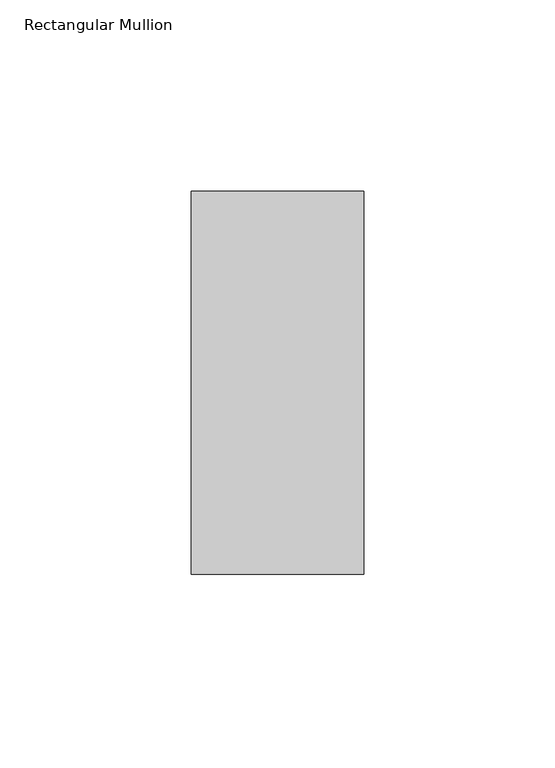
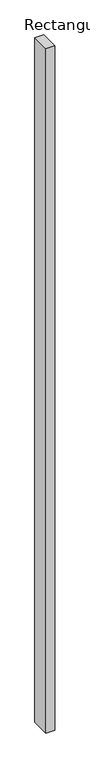
"""IFC4 building model written with IfcOpenShell, lengths in millimetres: member geometry, Rectangular Mullion : 알루미늄_Rectangular Cap_100 x 45."""

from ifc_helpers import new_model, si_unit, frame, origin, place, context, project, spatial, polyline, outline, extrude, source, transform, mapped, element, save


def rectangular_mullion_03c4161e(model_context):
    return source(origin(), model_context, "Body", "SweptSolid", [
        extrude(outline(polyline([(0.0, 50.0), (0.0, -50.0), (-45.0, -50.0), (-45.0, 50.0), (0.0, 50.0)])), frame((0.0, 0.0, -3775.0), z_axis=(0.0, 0.0, 1.0), x_axis=(1.0, 0.0, 0.0)), (0.0, 0.0, 1.0), 3775.0),
    ])


if __name__ == "__main__":
    model = new_model("IFC4")
    model_context = context("Model", 3, world=origin())
    ifc_project = project(units=[si_unit("LENGTHUNIT", "METRE", prefix="MILLI")], contexts=[model_context])
    site = spatial("IfcSite", under=ifc_project)
    building = spatial("IfcBuilding", under=site)
    placement = place(None, origin())
    rectangular_mullion_shape = rectangular_mullion_03c4161e(model_context)
    element("IfcMember", 1, ObjectType="Rectangular Mullion : 알루미늄_Rectangular Cap_100 x 45", at=placement, inside=building, context=model_context, shape_type="MappedRepresentation", body=[
        mapped(rectangular_mullion_shape, transform((0.0, 0.0, 0.0), x_axis=(1.0, 0.0, 0.0), y_axis=(0.0, 1.0, 0.0), z_axis=(0.0, 0.0, 1.0))),
    ])
    save(model, "model.ifc")

# Revit data of these elements
# Type "Rectangular Mullion : 알루미늄_Rectangular Cap_100 x 45"
#   built-in parameter 1007304 = 0.328084 (stored number, unit not read)
#   built-in parameter 1007301 = 0.0738189 (stored number, unit not read)
#   built-in parameter 1007300 = 0.0738189 (stored number, unit not read)
# Element 1 (IfcMember, "Rectangular Mullion : 알루미늄_Rectangular Cap_100 x 45")
#   Materials on its faces: "00_Metal_Stainless Steel"
# Materials
#   "00_Metal_Stainless Steel": class "Metal", colour RGB 148 148 148, transparency 0, Description = "Steel", Cost = 0
